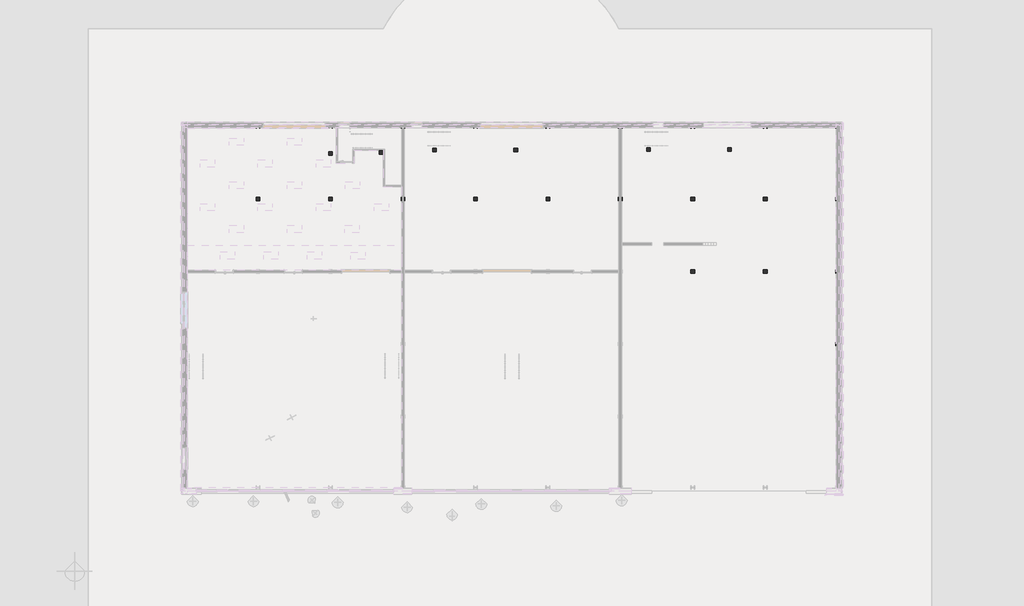
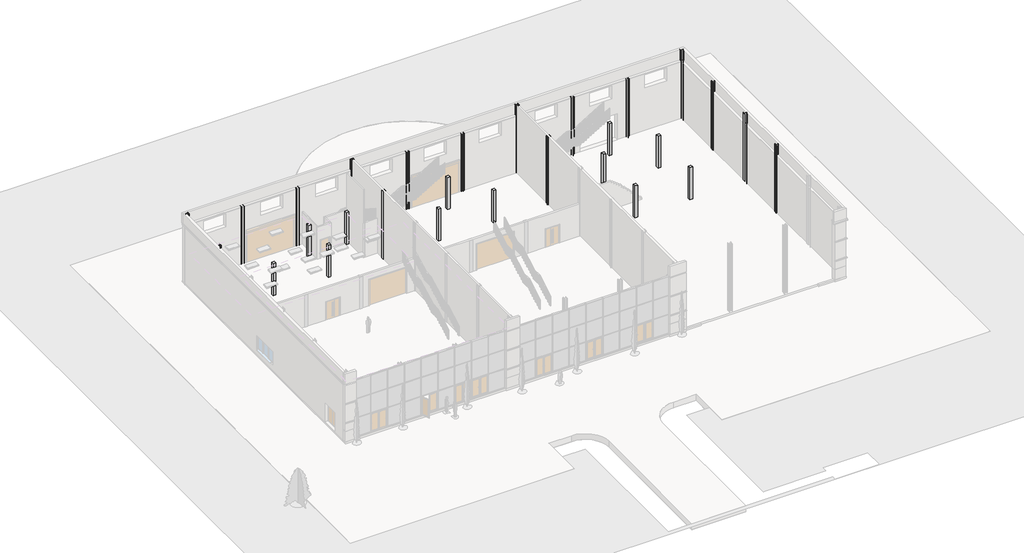
# One storey, part 6 of 13: 30 columns, 25 slabs, 2 footings.
"""IFC4 building model written with IfcOpenShell, lengths in millimetres."""

import ifcopenshell
import ifcopenshell.guid

model = None  # the IFC model being written
_history = None  # IfcOwnerHistory: only IFC2X3 demands one
_inside = {}  # id of a spatial element -> (the spatial element, [elements in it])
_under = {}  # id of a project, library or spatial element -> (it, [spatial elements below it])
_declared = {}  # id of a project -> (the project, [libraries it declares])
_typed = {}  # id of a type object -> (the type object, [elements of that type])
_made_of = {}  # id of a material, layer set ... -> (it, [elements and type objects made of it])


def new_model(schema):
    """Start an empty IFC model of exactly this schema.

    Asked for "IFC4X3", IfcOpenShell would pick the latest addendum, in which some entities
    have other attributes; the version numbers below select the first issue.
    IFC2X3 requires an IfcOwnerHistory on every rooted entity: one is made here for all.
    """
    global model, _history
    if schema == "IFC4X3":
        model = ifcopenshell.file(schema_version=(4, 3, 0, 0))
    else:
        model = ifcopenshell.file(schema=schema)
    _inside.clear()
    _under.clear()
    _declared.clear()
    _typed.clear()
    _made_of.clear()
    _history = None
    if model.schema == "IFC2X3":
        org = make("IfcOrganization", Name="unknown")
        user = make(
            "IfcPersonAndOrganization",
            ThePerson=make("IfcPerson", FamilyName="unknown"),
            TheOrganization=org,
        )
        app = make(
            "IfcApplication",
            ApplicationDeveloper=org,
            Version="unknown",
            ApplicationFullName="unknown",
            ApplicationIdentifier="unknown",
        )
        _history = make(
            "IfcOwnerHistory",
            OwningUser=user,
            OwningApplication=app,
            ChangeAction="ADDED",
            CreationDate=0,
        )
    return model


def make(cls, **values):
    """One entity of the class cls with the attributes given. An attribute that is None is left unset."""
    return model.create_entity(
        cls, **{name: value for name, value in values.items() if value is not None}
    )


def rooted(cls, **values):
    """An entity with a GlobalId (a new one), such as an element, a storey or a relation."""
    return make(cls, GlobalId=ifcopenshell.guid.new(), OwnerHistory=_history, **values)


def si_unit(unit_type, name, prefix=None):
    """IfcSIUnit, for example si_unit("LENGTHUNIT", "METRE", prefix="MILLI")."""
    return make("IfcSIUnit", UnitType=unit_type, Prefix=prefix, Name=name)


def assignment(units):
    """IfcUnitAssignment: the units of a project."""
    return None if units is None else make("IfcUnitAssignment", Units=units)


def point(xyz):
    """IfcCartesianPoint."""
    return None if xyz is None else make("IfcCartesianPoint", Coordinates=xyz)


def direction(xyz):
    """IfcDirection."""
    return None if xyz is None else make("IfcDirection", DirectionRatios=xyz)


def frame(location, z_axis=None, x_axis=None):
    """IfcAxis2Placement3D, a coordinate frame: its origin and axes. An axis left out is left unset."""
    return make(
        "IfcAxis2Placement3D",
        Location=point(location),
        Axis=direction(z_axis),
        RefDirection=direction(x_axis),
    )


def frame_2d(location, x_axis=None):
    """IfcAxis2Placement2D, a coordinate frame in the plane: its origin and x axis."""
    return make(
        "IfcAxis2Placement2D", Location=point(location), RefDirection=direction(x_axis)
    )


def origin():
    """The frame at (0, 0, 0) with its axes left unset."""
    return frame((0.0, 0.0, 0.0))


def place(relative_to, where):
    """IfcLocalPlacement: puts the frame where relative to a parent placement (None: the world)."""
    return make(
        "IfcLocalPlacement", PlacementRelTo=relative_to, RelativePlacement=where
    )


def context(
    kind, dimensions, precision=None, world=None, true_north=None, identifier=None
):
    """IfcGeometricRepresentationContext, for example the 3D "Model" context."""
    return make(
        "IfcGeometricRepresentationContext",
        ContextIdentifier=identifier,
        ContextType=kind,
        CoordinateSpaceDimension=dimensions,
        Precision=precision,
        WorldCoordinateSystem=world,
        TrueNorth=true_north,
    )


def project(units=None, contexts=None):
    """IfcProject with its units and contexts."""
    return rooted(
        "IfcProject",
        Name="project",
        RepresentationContexts=contexts,
        UnitsInContext=assignment(units),
    )


def spatial(cls, under=None, at=None, **own):
    """A site, building, storey or space (cls), placed at a placement, below another one or the project."""
    s = rooted(cls, ObjectPlacement=at, **own)
    if under is not None:
        _under.setdefault(under.id(), (under, []))[1].append(s)
    return s


def polyline(points):
    """IfcPolyline through the points."""
    return make("IfcPolyline", Points=[point(p) for p in points])


def circle_curve(where, radius):
    """IfcCircle in the frame where."""
    return make("IfcCircle", Position=where, Radius=radius)


def trimmed(basis, trim1, trim2, sense, master):
    """IfcTrimmedCurve: the piece of a basis curve between two trims."""
    return make(
        "IfcTrimmedCurve",
        BasisCurve=basis,
        Trim1=trim1,
        Trim2=trim2,
        SenseAgreement=sense,
        MasterRepresentation=master,
    )


def segment(curve, same_sense, transition):
    """IfcCompositeCurveSegment."""
    return make(
        "IfcCompositeCurveSegment",
        Transition=transition,
        SameSense=same_sense,
        ParentCurve=curve,
    )


def composite_curve(segments, self_intersect=None):
    """IfcCompositeCurve: segments joined end to end."""
    return make("IfcCompositeCurve", Segments=segments, SelfIntersect=self_intersect)


def outline(outer, holes=None, kind="AREA"):
    """IfcArbitraryClosedProfileDef: a profile drawn as a closed curve; with holes, ...WithVoids."""
    if holes is None:
        return make("IfcArbitraryClosedProfileDef", ProfileType=kind, OuterCurve=outer)
    return make(
        "IfcArbitraryProfileDefWithVoids",
        ProfileType=kind,
        OuterCurve=outer,
        InnerCurves=holes,
    )


def extrude(swept, where, along, depth):
    """IfcExtrudedAreaSolid: the profile swept, set in the frame where, extruded along a direction by depth."""
    return make(
        "IfcExtrudedAreaSolid",
        SweptArea=swept,
        Position=where,
        ExtrudedDirection=direction(along),
        Depth=depth,
    )


def faces_of(points, faces, orient=None, outer=None):
    """IfcFace entities. A face is a list of loops; a loop is a list of indices into points, from 0.

    orient and outer hold one flag for each loop. By default every Orientation is true, the
    first loop of a face is its IfcFaceOuterBound and the others are IfcFaceBound.
    """
    made = []
    for i, loops in enumerate(faces):
        bounds = []
        for j, loop in enumerate(loops):
            is_outer = j == 0 if outer is None else outer[i][j]
            bounds.append(
                make(
                    "IfcFaceOuterBound" if is_outer else "IfcFaceBound",
                    Bound=make("IfcPolyLoop", Polygon=[points[k] for k in loop]),
                    Orientation=True if orient is None else orient[i][j],
                )
            )
        made.append(make("IfcFace", Bounds=bounds))
    return made


def faceted_brep(points, faces, orient=None, outer=None, voids=None):
    """IfcFacetedBrep: a solid bounded by flat faces; with voids (closed shells), ...WithVoids."""
    shared = [point(p) for p in points]
    hull = make("IfcClosedShell", CfsFaces=faces_of(shared, faces, orient, outer))
    if voids is None:
        return make("IfcFacetedBrep", Outer=hull)
    return make(
        "IfcFacetedBrepWithVoids",
        Outer=hull,
        Voids=[
            make(cls, CfsFaces=faces_of(shared, fs, o, b)) for cls, fs, o, b in voids
        ],
    )


def shape(context_of_items, identifier, shape_type, items):
    """IfcShapeRepresentation: the items that make up one representation, for example the "Body"."""
    return make(
        "IfcShapeRepresentation",
        ContextOfItems=context_of_items,
        RepresentationIdentifier=identifier,
        RepresentationType=shape_type,
        Items=items,
    )


def source(mapping_origin, context_of_items, identifier, shape_type, items):
    """IfcRepresentationMap: a shape defined once, which mapped items show again and again."""
    return make(
        "IfcRepresentationMap",
        MappingOrigin=mapping_origin,
        MappedRepresentation=shape(context_of_items, identifier, shape_type, items),
    )


def transform(
    local_origin,
    x_axis=None,
    y_axis=None,
    z_axis=None,
    scale=None,
    scale2=None,
    scale3=None,
    uniform=True,
):
    """IfcCartesianTransformationOperator3D, or its non-uniform kind. x_axis, y_axis, z_axis: its Axis1, 2, 3."""
    if uniform:
        return make(
            "IfcCartesianTransformationOperator3D",
            Axis1=direction(x_axis),
            Axis2=direction(y_axis),
            LocalOrigin=point(local_origin),
            Scale=scale,
            Axis3=direction(z_axis),
        )
    return make(
        "IfcCartesianTransformationOperator3DnonUniform",
        Axis1=direction(x_axis),
        Axis2=direction(y_axis),
        LocalOrigin=point(local_origin),
        Scale=scale,
        Axis3=direction(z_axis),
        Scale2=scale2,
        Scale3=scale3,
    )


def mapped(mapping_source, mapping_target):
    """IfcMappedItem: shows the shape of a source again, moved by a transform."""
    return make(
        "IfcMappedItem", MappingSource=mapping_source, MappingTarget=mapping_target
    )


def made_of(thing, what):
    """Note that an element or type object is made of a material, layer set ...; save() writes the relation."""
    if what is not None:
        _made_of.setdefault(what.id(), (what, []))[1].append(thing)
    return thing


def element(
    cls,
    number,
    at=None,
    inside=None,
    cuts=None,
    type_object=None,
    material=None,
    context=None,
    identifier="Body",
    shape_type=None,
    held_by="IfcProductDefinitionShape",
    body=None,
    shapes=None,
    **own,
):
    """One element of the class cls, such as IfcWall. Its Tag is "e" and its number.

    at: its placement. inside: the storey or other place that contains it. cuts: it is an
    opening in that element (IfcRelVoidsElement). A single representation is given by context,
    identifier, shape_type and body (its items); several are given by shapes. held_by: the class
    of the entity that holds the representations. save() writes the other relations.
    """
    e = rooted(cls, Tag="e%d" % number, ObjectPlacement=at, **own)
    if body is not None:
        shapes = [shape(context, identifier, shape_type, body)]
    if shapes is not None:
        e.Representation = make(held_by, Representations=shapes)
    if inside is not None:
        _inside.setdefault(inside.id(), (inside, []))[1].append(e)
    if cuts is not None:
        rooted(
            "IfcRelVoidsElement", RelatingBuildingElement=cuts, RelatedOpeningElement=e
        )
    if type_object is not None:
        _typed.setdefault(type_object.id(), (type_object, []))[1].append(e)
    return made_of(e, material)


def aggregate(whole, parts):
    """IfcRelAggregates: a whole, such as a stair, and the parts it consists of."""
    return rooted("IfcRelAggregates", RelatingObject=whole, RelatedObjects=parts)


def save(model, path):
    """Write the relations noted so far, then the file.

    IfcRelAggregates (storeys below a building ...), IfcRelContainedInSpatialStructure (elements
    in a storey), IfcRelDefinesByType, IfcRelAssociatesMaterial and IfcRelDeclares: one each for
    every whole, place, type object, material and project.
    """
    for whole, parts in _under.values():
        aggregate(whole, parts)
    for where, things in _inside.values():
        rooted(
            "IfcRelContainedInSpatialStructure",
            RelatedElements=things,
            RelatingStructure=where,
        )
    for kind, things in _typed.values():
        rooted("IfcRelDefinesByType", RelatedObjects=things, RelatingType=kind)
    for what, things in _made_of.values():
        rooted("IfcRelAssociatesMaterial", RelatedObjects=things, RelatingMaterial=what)
    for by, libraries in _declared.values():
        rooted("IfcRelDeclares", RelatingContext=by, RelatedDefinitions=libraries)
    model.write(path)


def uc_universal_column_column_305x305x97uc_f4bfb62a(model_context):
    return source(origin(), model_context, "Body", "SweptSolid", [
        extrude(outline(composite_curve([segment(polyline([(152.65, 153.95), (152.65, 138.55), (20.15, 138.55)]), True, "CONTINUOUS"), segment(trimmed(circle_curve(frame_2d((20.15, 123.35)), 15.2), [point((20.15, 138.55))], [point((4.95, 123.35))], True, "CARTESIAN"), True, "CONTINUOUS"), segment(polyline([(4.95, 123.35), (4.95, -123.35)]), True, "CONTINUOUS"), segment(trimmed(circle_curve(frame_2d((20.15, -123.35)), 15.2), [point((4.95, -123.35))], [point((20.15, -138.55))], True, "CARTESIAN"), True, "CONTINUOUS"), segment(polyline([(20.15, -138.55), (152.65, -138.55), (152.65, -153.95), (-152.65, -153.95), (-152.65, -138.55), (-20.15, -138.55)]), True, "CONTINUOUS"), segment(trimmed(circle_curve(frame_2d((-20.15, -123.35)), 15.2), [point((-20.15, -138.55))], [point((-4.95, -123.35))], True, "CARTESIAN"), True, "CONTINUOUS"), segment(polyline([(-4.95, -123.35), (-4.95, 123.35)]), True, "CONTINUOUS"), segment(trimmed(circle_curve(frame_2d((-20.15, 123.35)), 15.2), [point((-4.95, 123.35))], [point((-20.15, 138.55))], True, "CARTESIAN"), True, "CONTINUOUS"), segment(polyline([(-20.15, 138.55), (-152.65, 138.55), (-152.65, 153.95), (152.65, 153.95)]), True, "CONTINUOUS")], self_intersect=False)), frame((0.0, 0.0, -1500.0), z_axis=(0.0, 0.0, 1.0), x_axis=(1.0, 0.0, 0.0)), (0.0, 0.0, 1.0), 9300.0),
    ])


def uc_universal_column_column_305x305x97uc_8da79b43(model_context):
    return source(origin(), model_context, "Body", "SweptSolid", [
        extrude(outline(composite_curve([segment(polyline([(152.65, -153.95), (-152.65, -153.95), (-152.65, -138.55), (-20.15, -138.55)]), True, "CONTINUOUS"), segment(trimmed(circle_curve(frame_2d((-20.15, -123.35)), 15.2), [point((-20.15, -138.55))], [point((-4.95, -123.35))], True, "CARTESIAN"), True, "CONTINUOUS"), segment(polyline([(-4.95, -123.35), (-4.95, 123.35)]), True, "CONTINUOUS"), segment(trimmed(circle_curve(frame_2d((-20.15, 123.35)), 15.2), [point((-4.95, 123.35))], [point((-20.15, 138.55))], True, "CARTESIAN"), True, "CONTINUOUS"), segment(polyline([(-20.15, 138.55), (-152.65, 138.55), (-152.65, 153.95), (152.65, 153.95), (152.65, 138.55), (20.15, 138.55)]), True, "CONTINUOUS"), segment(trimmed(circle_curve(frame_2d((20.15, 123.35)), 15.2), [point((20.15, 138.55))], [point((4.95, 123.35))], True, "CARTESIAN"), True, "CONTINUOUS"), segment(polyline([(4.95, 123.35), (4.95, -123.35)]), True, "CONTINUOUS"), segment(trimmed(circle_curve(frame_2d((20.15, -123.35)), 15.2), [point((4.95, -123.35))], [point((20.15, -138.55))], True, "CARTESIAN"), True, "CONTINUOUS"), segment(polyline([(20.15, -138.55), (152.65, -138.55), (152.65, -153.95)]), True, "CONTINUOUS")], self_intersect=False)), frame((0.0, 0.0, -1500.0), z_axis=(0.0, 0.0, 1.0), x_axis=(1.0, 0.0, 0.0)), (0.0, 0.0, 1.0), 9300.0),
    ])


def uc_universal_column_column_305x305x97uc_43a052ce(model_context):
    return source(origin(), model_context, "Body", "SweptSolid", [
        extrude(outline(composite_curve([segment(polyline([(152.65, 153.95), (152.65, 138.55), (20.15, 138.55)]), True, "CONTINUOUS"), segment(trimmed(circle_curve(frame_2d((20.15, 123.35)), 15.2), [point((20.15, 138.55))], [point((4.95, 123.35))], True, "CARTESIAN"), True, "CONTINUOUS"), segment(polyline([(4.95, 123.35), (4.95, -123.35)]), True, "CONTINUOUS"), segment(trimmed(circle_curve(frame_2d((20.15, -123.35)), 15.2), [point((4.95, -123.35))], [point((20.15, -138.55))], True, "CARTESIAN"), True, "CONTINUOUS"), segment(polyline([(20.15, -138.55), (152.65, -138.55), (152.65, -153.95), (-152.65, -153.95), (-152.65, -138.55), (-20.15, -138.55)]), True, "CONTINUOUS"), segment(trimmed(circle_curve(frame_2d((-20.15, -123.35)), 15.2), [point((-20.15, -138.55))], [point((-4.95, -123.35))], True, "CARTESIAN"), True, "CONTINUOUS"), segment(polyline([(-4.95, -123.35), (-4.95, 123.35)]), True, "CONTINUOUS"), segment(trimmed(circle_curve(frame_2d((-20.15, 123.35)), 15.2), [point((-4.95, 123.35))], [point((-20.15, 138.55))], True, "CARTESIAN"), True, "CONTINUOUS"), segment(polyline([(-20.15, 138.55), (-152.65, 138.55), (-152.65, 153.95), (152.65, 153.95)]), True, "CONTINUOUS")], self_intersect=False)), frame((0.0, 0.0, -1500.0), z_axis=(0.0, 0.0, 1.0), x_axis=(1.0, 0.0, 0.0)), (0.0, 0.0, 1.0), 8100.0),
    ])


def pad_foundation_rectangular_1000x1000x500_ed6229e9(model_context):
    return source(origin(), model_context, "Body", "SweptSolid", [
        extrude(outline(polyline([(500.0, 500.0), (500.0, -500.0), (-500.0, -500.0), (-500.0, 500.0), (500.0, 500.0)])), frame((0.0, 0.0, -500.0), z_axis=(0.0, 0.0, 1.0), x_axis=(1.0, 0.0, 0.0)), (0.0, 0.0, 1.0), 500.0),
    ])


model = new_model("IFC4")

# Units and contexts
model_context = context("Model", 3, world=origin())
ifc_project = project(units=[si_unit("LENGTHUNIT", "METRE", prefix="MILLI")], contexts=[model_context])

# Site, building, storey
site = spatial("IfcSite", under=ifc_project)
building = spatial("IfcBuilding", under=site)
storey = spatial("IfcBuildingStorey", under=building, Name="L0 - Ground Floor (Shadows On)", Elevation=0.0)

# Columns
placement = place(None, origin())
element("IfcColumn", 1, ObjectType="Concrete Square : 300 x 300mm", at=placement, inside=storey, context=model_context, shape_type="SweptSolid", body=[
    extrude(outline(polyline([(-989.5553457, 791.2380918), (-1289.5553457, 791.2380918), (-1289.5553457, 1091.2380918), (-989.5553457, 1091.2380918), (-989.5553457, 791.2380918)])), frame((0.0, 0.0, -1500.0), z_axis=(0.0, 0.0, 1.0), x_axis=(1.0, 0.0, 0.0)), (0.0, 0.0, 1.0), 5200.0),
])
element("IfcColumn", 2, ObjectType="Concrete Square : 300 x 300mm", at=placement, inside=storey, context=model_context, shape_type="SweptSolid", body=[
    extrude(outline(polyline([(9194.5066977, 4635.3001351), (8894.5066977, 4635.3001351), (8894.5066977, 4935.3001351), (9194.5066977, 4935.3001351), (9194.5066977, 4635.3001351)])), frame((0.0, 0.0, -1500.0), z_axis=(0.0, 0.0, 1.0), x_axis=(1.0, 0.0, 0.0)), (0.0, 0.0, 1.0), 5200.0),
])
element("IfcColumn", 3, ObjectType="Concrete Square : 300 x 300mm", at=placement, inside=storey, context=model_context, shape_type="SweptSolid", body=[
    extrude(outline(polyline([(17010.4446543, 791.2380918), (16710.4446543, 791.2380918), (16710.4446543, 1091.2380918), (17010.4446543, 1091.2380918), (17010.4446543, 791.2380918)])), frame((0.0, 0.0, -1500.0), z_axis=(0.0, 0.0, 1.0), x_axis=(1.0, 0.0, 0.0)), (0.0, 0.0, 1.0), 5200.0),
])
element("IfcColumn", 4, ObjectType="Concrete Square : 300 x 300mm", at=placement, inside=storey, context=model_context, shape_type="SweptSolid", body=[
    extrude(outline(polyline([(23010.4446543, 791.2380918), (22710.4446543, 791.2380918), (22710.4446543, 1091.2380918), (23010.4446543, 1091.2380918), (23010.4446543, 791.2380918)])), frame((0.0, 0.0, -1500.0), z_axis=(0.0, 0.0, 1.0), x_axis=(1.0, 0.0, 0.0)), (0.0, 0.0, 1.0), 5200.0),
])
element("IfcColumn", 5, ObjectType="Concrete Square : 300 x 300mm", at=placement, inside=storey, context=model_context, shape_type="SweptSolid", body=[
    extrude(outline(polyline([(35010.4446543, 791.2380918), (34710.4446543, 791.2380918), (34710.4446543, 1091.2380918), (35010.4446543, 1091.2380918), (35010.4446543, 791.2380918)])), frame((0.0, 0.0, -1500.0), z_axis=(0.0, 0.0, 1.0), x_axis=(1.0, 0.0, 0.0)), (0.0, 0.0, 1.0), 5200.0),
])
element("IfcColumn", 6, ObjectType="Concrete Square : 300 x 300mm", at=placement, inside=storey, context=model_context, shape_type="SweptSolid", body=[
    extrude(outline(polyline([(41010.4446543, 791.2380918), (40710.4446543, 791.2380918), (40710.4446543, 1091.2380918), (41010.4446543, 1091.2380918), (41010.4446543, 791.2380918)])), frame((0.0, 0.0, -1500.0), z_axis=(0.0, 0.0, 1.0), x_axis=(1.0, 0.0, 0.0)), (0.0, 0.0, 1.0), 5200.0),
])
element("IfcColumn", 7, ObjectType="Concrete Square : 300 x 300mm", at=placement, inside=storey, context=model_context, shape_type="SweptSolid", body=[
    extrude(outline(polyline([(35010.4446543, -5208.7619082), (34710.4446543, -5208.7619082), (34710.4446543, -4908.7619082), (35010.4446543, -4908.7619082), (35010.4446543, -5208.7619082)])), frame((0.0, 0.0, -1500.0), z_axis=(0.0, 0.0, 1.0), x_axis=(1.0, 0.0, 0.0)), (0.0, 0.0, 1.0), 5200.0),
])
element("IfcColumn", 8, ObjectType="Concrete Square : 300 x 300mm", at=placement, inside=storey, context=model_context, shape_type="SweptSolid", body=[
    extrude(outline(polyline([(41010.4446543, -5208.7619082), (40710.4446543, -5208.7619082), (40710.4446543, -4908.7619082), (41010.4446543, -4908.7619082), (41010.4446543, -5208.7619082)])), frame((0.0, 0.0, -1500.0), z_axis=(0.0, 0.0, 1.0), x_axis=(1.0, 0.0, 0.0)), (0.0, 0.0, 1.0), 5200.0),
])
element("IfcColumn", 9, ObjectType="Concrete Square : 300 x 300mm", at=placement, inside=storey, context=model_context, shape_type="SweptSolid", body=[
    extrude(outline(polyline([(5010.4446543, 791.2380918), (4710.4446543, 791.2380918), (4710.4446543, 1091.2380918), (5010.4446543, 1091.2380918), (5010.4446543, 791.2380918)])), frame((0.0, 0.0, -1500.0), z_axis=(0.0, 0.0, 1.0), x_axis=(1.0, 0.0, 0.0)), (0.0, 0.0, 1.0), 5200.0),
])
element("IfcColumn", 10, ObjectType="Concrete Square : 300 x 300mm", at=placement, inside=storey, context=model_context, shape_type="SweptSolid", body=[
    extrude(outline(polyline([(5022.9446543, 4575.3001351), (4722.9446543, 4575.3001351), (4722.9446543, 4875.3001351), (5022.9446543, 4875.3001351), (5022.9446543, 4575.3001351)])), frame((0.0, 0.0, -1500.0), z_axis=(0.0, 0.0, 1.0), x_axis=(1.0, 0.0, 0.0)), (0.0, 0.0, 1.0), 5200.0),
])
element("IfcColumn", 11, ObjectType="Concrete Square : 300 x 300mm", at=placement, inside=storey, context=model_context, shape_type="SweptSolid", body=[
    extrude(outline(polyline([(20350.4446543, 4850.3001351), (20050.4446543, 4850.3001351), (20050.4446543, 5150.3001351), (20350.4446543, 5150.3001351), (20350.4446543, 4850.3001351)])), frame((0.0, 0.0, -1500.0), z_axis=(0.0, 0.0, 1.0), x_axis=(1.0, 0.0, 0.0)), (0.0, 0.0, 1.0), 5200.0),
])
element("IfcColumn", 12, ObjectType="Concrete Square : 300 x 300mm", at=placement, inside=storey, context=model_context, shape_type="SweptSolid", body=[
    extrude(outline(polyline([(13627.9446543, 5150.3001351), (13627.9446543, 4850.3001351), (13327.9446543, 4850.3001351), (13327.9446543, 5150.3001351), (13627.9446543, 5150.3001351)])), frame((0.0, 0.0, -1500.0), z_axis=(0.0, 0.0, 1.0), x_axis=(1.0, 0.0, 0.0)), (0.0, 0.0, 1.0), 5200.0),
])
element("IfcColumn", 13, ObjectType="Concrete Square : 300 x 300mm", at=placement, inside=storey, context=model_context, shape_type="SweptSolid", body=[
    extrude(outline(polyline([(31350.4446543, 4891.2380918), (31050.4446543, 4891.2380918), (31050.4446543, 5191.2380918), (31350.4446543, 5191.2380918), (31350.4446543, 4891.2380918)])), frame((0.0, 0.0, -1500.0), z_axis=(0.0, 0.0, 1.0), x_axis=(1.0, 0.0, 0.0)), (0.0, 0.0, 1.0), 5200.0),
])
element("IfcColumn", 14, ObjectType="Concrete Square : 300 x 300mm", at=placement, inside=storey, context=model_context, shape_type="SweptSolid", body=[
    extrude(outline(polyline([(38050.4446543, 4891.2380918), (37750.4446543, 4891.2380918), (37750.4446543, 5191.2380918), (38050.4446543, 5191.2380918), (38050.4446543, 4891.2380918)])), frame((0.0, 0.0, -1500.0), z_axis=(0.0, 0.0, 1.0), x_axis=(1.0, 0.0, 0.0)), (0.0, 0.0, 1.0), 5200.0),
])
element("IfcColumn", 15, ObjectType="UC-Universal Column-Column : 305x305x97UC", at=placement, inside=storey, context=model_context, shape_type="SweptSolid", body=[
    extrude(outline(composite_curve([segment(polyline([(-7293.5053457, 1093.8880918), (-7278.1053457, 1093.8880918), (-7278.1053457, 961.3880918)]), True, "CONTINUOUS"), segment(trimmed(circle_curve(frame_2d((-7262.9053457, 961.3880918)), 15.2), [point((-7278.1053457, 961.3880918))], [point((-7262.9053457, 946.1880918))], True, "CARTESIAN"), True, "CONTINUOUS"), segment(polyline([(-7262.9053457, 946.1880918), (-7016.2053457, 946.1880918)]), True, "CONTINUOUS"), segment(trimmed(circle_curve(frame_2d((-7016.2053457, 961.3880918)), 15.2), [point((-7016.2053457, 946.1880918))], [point((-7001.0053457, 961.3880918))], True, "CARTESIAN"), True, "CONTINUOUS"), segment(polyline([(-7001.0053457, 961.3880918), (-7001.0053457, 1093.8880918), (-6985.6053457, 1093.8880918), (-6985.6053457, 788.5880918), (-7001.0053457, 788.5880918), (-7001.0053457, 921.0880918)]), True, "CONTINUOUS"), segment(trimmed(circle_curve(frame_2d((-7016.2053457, 921.0880918)), 15.2), [point((-7001.0053457, 921.0880918))], [point((-7016.2053457, 936.2880918))], True, "CARTESIAN"), True, "CONTINUOUS"), segment(polyline([(-7016.2053457, 936.2880918), (-7262.9053457, 936.2880918)]), True, "CONTINUOUS"), segment(trimmed(circle_curve(frame_2d((-7262.9053457, 921.0880918)), 15.2), [point((-7262.9053457, 936.2880918))], [point((-7278.1053457, 921.0880918))], True, "CARTESIAN"), True, "CONTINUOUS"), segment(polyline([(-7278.1053457, 921.0880918), (-7278.1053457, 788.5880918), (-7293.5053457, 788.5880918), (-7293.5053457, 1093.8880918)]), True, "CONTINUOUS")], self_intersect=False)), frame((0.0, 0.0, -1500.0), z_axis=(0.0, 0.0, 1.0), x_axis=(1.0, 0.0, 0.0)), (0.0, 0.0, 1.0), 9300.0),
])
uc_universal_column_column_305x305x97uc_shape = uc_universal_column_column_305x305x97uc_f4bfb62a(model_context)
element("IfcColumn", 16, ObjectType="UC-Universal Column-Column : 305x305x97UC", at=placement, inside=storey, context=model_context, shape_type="MappedRepresentation", body=[
    mapped(uc_universal_column_column_305x305x97uc_shape, transform((-7139.5553457, 6941.2380918, 0.0), x_axis=(0.0, 1.0, 0.0), y_axis=(-1.0, 0.0, 0.0), z_axis=(0.0, 0.0, 1.0))),
])
element("IfcColumn", 17, ObjectType="UC-Universal Column-Column : 305x305x97UC", at=placement, inside=storey, context=model_context, shape_type="MappedRepresentation", body=[
    mapped(uc_universal_column_column_305x305x97uc_shape, transform((10860.4446543, 6941.2380918, 0.0), x_axis=(0.0, 1.0, 0.0), y_axis=(-1.0, 0.0, 0.0), z_axis=(0.0, 0.0, 1.0))),
])
element("IfcColumn", 18, ObjectType="UC-Universal Column-Column : 305x305x97UC", at=placement, inside=storey, context=model_context, shape_type="MappedRepresentation", body=[
    mapped(uc_universal_column_column_305x305x97uc_shape, transform((28860.4446543, 6941.2380918, 0.0), x_axis=(0.0, 1.0, 0.0), y_axis=(-1.0, 0.0, 0.0), z_axis=(0.0, 0.0, 1.0))),
])
element("IfcColumn", 19, ObjectType="UC-Universal Column-Column : 305x305x97UC", at=placement, inside=storey, context=model_context, shape_type="MappedRepresentation", body=[
    mapped(uc_universal_column_column_305x305x97uc_shape, transform((10860.4446543, 941.2380918, 0.0), x_axis=(0.0, 1.0, 0.0), y_axis=(-1.0, 0.0, 0.0), z_axis=(0.0, 0.0, 1.0))),
])
element("IfcColumn", 20, ObjectType="UC-Universal Column-Column : 305x305x97UC", at=placement, inside=storey, context=model_context, shape_type="MappedRepresentation", body=[
    mapped(uc_universal_column_column_305x305x97uc_shape, transform((28860.4446543, 941.2380918, 0.0), x_axis=(0.0, 1.0, 0.0), y_axis=(-1.0, 0.0, 0.0), z_axis=(0.0, 0.0, 1.0))),
])
uc_universal_column_column_305x305x97uc_2_shape = uc_universal_column_column_305x305x97uc_8da79b43(model_context)
element("IfcColumn", 21, ObjectType="UC-Universal Column-Column : 305x305x97UC", at=placement, inside=storey, context=model_context, shape_type="MappedRepresentation", body=[
    mapped(uc_universal_column_column_305x305x97uc_2_shape, transform((46860.4446543, -11058.7619082, 0.0), x_axis=(0.0, 1.0, 0.0), y_axis=(-1.0, 0.0, 0.0), z_axis=(0.0, 0.0, 1.0))),
])
element("IfcColumn", 22, ObjectType="UC-Universal Column-Column : 305x305x97UC", at=placement, inside=storey, context=model_context, shape_type="MappedRepresentation", body=[
    mapped(uc_universal_column_column_305x305x97uc_2_shape, transform((46860.4446543, -5058.7619082, 0.0), x_axis=(0.0, 1.0, 0.0), y_axis=(-1.0, 0.0, 0.0), z_axis=(0.0, 0.0, 1.0))),
])
element("IfcColumn", 23, ObjectType="UC-Universal Column-Column : 305x305x97UC", at=placement, inside=storey, context=model_context, shape_type="MappedRepresentation", body=[
    mapped(uc_universal_column_column_305x305x97uc_2_shape, transform((46860.4446543, 941.2380918, 0.0), x_axis=(0.0, 1.0, 0.0), y_axis=(-1.0, 0.0, 0.0), z_axis=(0.0, 0.0, 1.0))),
])
element("IfcColumn", 24, ObjectType="UC-Universal Column-Column : 305x305x97UC", at=placement, inside=storey, context=model_context, shape_type="MappedRepresentation", body=[
    mapped(uc_universal_column_column_305x305x97uc_2_shape, transform((46860.4446543, 6941.2380918, 0.0), x_axis=(0.0, 1.0, 0.0), y_axis=(-1.0, 0.0, 0.0), z_axis=(0.0, 0.0, 1.0))),
])
uc_universal_column_column_305x305x97uc_3_shape = uc_universal_column_column_305x305x97uc_43a052ce(model_context)
element("IfcColumn", 25, ObjectType="UC-Universal Column-Column : 305x305x97UC", at=placement, inside=storey, context=model_context, shape_type="MappedRepresentation", body=[
    mapped(uc_universal_column_column_305x305x97uc_3_shape, transform((-1139.5553457, 6941.2380918, 0.0), x_axis=(0.0, 1.0, 0.0), y_axis=(-1.0, 0.0, 0.0), z_axis=(0.0, 0.0, 1.0))),
])
element("IfcColumn", 26, ObjectType="UC-Universal Column-Column : 305x305x97UC", at=placement, inside=storey, context=model_context, shape_type="MappedRepresentation", body=[
    mapped(uc_universal_column_column_305x305x97uc_3_shape, transform((4860.4446543, 6941.2380918, 0.0), x_axis=(0.0, 1.0, 0.0), y_axis=(-1.0, 0.0, 0.0), z_axis=(0.0, 0.0, 1.0))),
])
element("IfcColumn", 27, ObjectType="UC-Universal Column-Column : 305x305x97UC", at=placement, inside=storey, context=model_context, shape_type="MappedRepresentation", body=[
    mapped(uc_universal_column_column_305x305x97uc_3_shape, transform((16860.4446543, 6941.2380918, 0.0), x_axis=(0.0, 1.0, 0.0), y_axis=(-1.0, 0.0, 0.0), z_axis=(0.0, 0.0, 1.0))),
])
element("IfcColumn", 28, ObjectType="UC-Universal Column-Column : 305x305x97UC", at=placement, inside=storey, context=model_context, shape_type="MappedRepresentation", body=[
    mapped(uc_universal_column_column_305x305x97uc_3_shape, transform((22860.4446543, 6941.2380918, 0.0), x_axis=(0.0, 1.0, 0.0), y_axis=(-1.0, 0.0, 0.0), z_axis=(0.0, 0.0, 1.0))),
])
element("IfcColumn", 29, ObjectType="UC-Universal Column-Column : 305x305x97UC", at=placement, inside=storey, context=model_context, shape_type="MappedRepresentation", body=[
    mapped(uc_universal_column_column_305x305x97uc_3_shape, transform((34860.4446543, 6941.2380918, 0.0), x_axis=(0.0, 1.0, 0.0), y_axis=(-1.0, 0.0, 0.0), z_axis=(0.0, 0.0, 1.0))),
])
element("IfcColumn", 30, ObjectType="UC-Universal Column-Column : 305x305x97UC", at=placement, inside=storey, context=model_context, shape_type="MappedRepresentation", body=[
    mapped(uc_universal_column_column_305x305x97uc_3_shape, transform((40860.4446543, 6941.2380918, 0.0), x_axis=(0.0, 1.0, 0.0), y_axis=(-1.0, 0.0, 0.0), z_axis=(0.0, 0.0, 1.0))),
])

# Footings
element("IfcFooting", 31, ObjectType="Wall Foundation - Commercial 1300 x 450", at=placement, inside=storey, context=model_context, shape_type="Brep", body=[
    faceted_brep([(47425.1446543, 7505.9380918, -1200.0), (46510.7446543, 7505.9380918, -1200.0), (46510.7446543, 6591.5380918, -1200.0), (46510.7446543, -22819.0474846, -1200.0), (47425.1446543, -22819.0474846, -1200.0), (47425.1446543, 7505.9380918, -1504.8), (47425.1446543, -22819.0474846, -1504.8), (46510.7446543, 7505.9380918, -1504.8), (47360.4446543, -22819.0474846, -1504.8), (47360.4446543, -22448.7619082, -1504.8), (46510.7446543, -22448.7619082, -1504.8), (46510.7446543, -17558.7619082, -1504.8), (47360.4446543, -17558.7619082, -1504.8), (47360.4446543, -16558.7619082, -1504.8), (46510.7446543, -16558.7619082, -1504.8), (46510.7446543, -11558.7619082, -1504.8), (47360.4446543, -11558.7619082, -1504.8), (47360.4446543, -10558.7619082, -1504.8), (46510.7446543, -10558.7619082, -1504.8), (46510.7446543, -5558.7619082, -1504.8), (47360.4446543, -5558.7619082, -1504.8), (47360.4446543, -4558.7619082, -1504.8), (46510.7446543, -4558.7619082, -1504.8), (46510.7446543, 441.2380918, -1504.8), (47360.4446543, 441.2380918, -1504.8), (47360.4446543, 1441.2380918, -1504.8), (46510.7446543, 1441.2380918, -1504.8), (46510.7446543, 6441.2380918, -1504.8), (47360.4446543, 6441.2380918, -1504.8), (47360.4446543, 7441.2380918, -1504.8), (46510.7446543, 7441.2380918, -1504.8), (46510.7446543, 7441.2380918, -1500.0), (46510.7446543, 6591.5380918, -1500.0), (46510.7446543, 6441.2380918, -1500.0), (46510.7446543, 1441.2380918, -1500.0), (46510.7446543, 441.2380918, -1500.0), (46510.7446543, -4558.7619082, -1500.0), (46510.7446543, -5558.7619082, -1500.0), (46510.7446543, -10558.7619082, -1500.0), (46510.7446543, -11558.7619082, -1500.0), (46510.7446543, -16558.7619082, -1500.0), (46510.7446543, -17558.7619082, -1500.0), (46510.7446543, -22448.7619082, -1500.0), (46510.7446543, -22819.0474846, -1500.0), (47360.4446543, 1441.2380918, -1500.0), (47360.4446543, 441.2380918, -1500.0), (47360.4446543, 7441.2380918, -1500.0), (47360.4446543, 6441.2380918, -1500.0), (47360.4446543, -4558.7619082, -1500.0), (47360.4446543, -5558.7619082, -1500.0), (47360.4446543, -10558.7619082, -1500.0), (47360.4446543, -11558.7619082, -1500.0), (47360.4446543, -16558.7619082, -1500.0), (47360.4446543, -17558.7619082, -1500.0), (47360.4446543, -22448.7619082, -1500.0), (47360.4446543, -22819.0474846, -1500.0)], [[[0, 1, 2, 3, 4]], [[5, 0, 4, 6]], [[7, 5, 6, 8, 9, 10, 11, 12, 13, 14, 15, 16, 17, 18, 19, 20, 21, 22, 23, 24, 25, 26, 27, 28, 29, 30]], [[1, 7, 30, 31, 32, 33, 27, 26, 34, 35, 23, 22, 36, 37, 19, 18, 38, 39, 15, 14, 40, 41, 11, 10, 42, 43, 3, 2]], [[1, 0, 5, 7]], [[44, 45, 35, 34]], [[44, 34, 26, 25]], [[35, 45, 24, 23]], [[45, 44, 25, 24]], [[46, 47, 33, 32, 31]], [[33, 47, 28, 27]], [[47, 46, 29, 28]], [[48, 49, 37, 36]], [[48, 36, 22, 21]], [[37, 49, 20, 19]], [[49, 48, 21, 20]], [[50, 51, 39, 38]], [[50, 38, 18, 17]], [[39, 51, 16, 15]], [[51, 50, 17, 16]], [[52, 53, 41, 40]], [[52, 40, 14, 13]], [[41, 53, 12, 11]], [[53, 52, 13, 12]], [[42, 54, 55, 43]], [[54, 42, 10, 9]], [[54, 9, 8, 55]], [[4, 3, 43, 55, 8, 6]], [[46, 31, 30, 29]]]),
])
element("IfcFooting", 32, ObjectType="Wall Foundation - Commercial 1300 x 450", at=placement, inside=storey, context=model_context, shape_type="Brep", body=[
    faceted_brep([(46510.7446543, 6591.5380918, -1200.0), (46510.7446543, 7505.9380918, -1200.0), (-6758.8053457, 7505.9380918, -1200.0), (-6758.8053457, 6591.5380918, -1200.0), (10403.2446543, 6591.5380918, -1200.0), (11317.6446543, 6591.5380918, -1200.0), (28403.2446543, 6591.5380918, -1200.0), (29317.6446543, 6591.5380918, -1200.0), (46510.7446543, 7505.9380918, -1504.8), (-6758.8053457, 7505.9380918, -1504.8), (41386.4946543, 7441.2380918, -1504.8), (40386.4946543, 7441.2380918, -1504.8), (40386.4946543, 6591.5380918, -1504.8), (35347.9446543, 6591.5380918, -1504.8), (35347.9446543, 7441.2380918, -1504.8), (34347.9446543, 7441.2380918, -1504.8), (34347.9446543, 6591.5380918, -1504.8), (29360.4446543, 6591.5380918, -1504.8), (29360.4446543, 7441.2380918, -1504.8), (28360.4446543, 7441.2380918, -1504.8), (28360.4446543, 6591.5380918, -1504.8), (23360.4446543, 6591.5380918, -1504.8), (23360.4446543, 7441.2380918, -1504.8), (22360.4446543, 7441.2380918, -1504.8), (22360.4446543, 6591.5380918, -1504.8), (17360.4446543, 6591.5380918, -1504.8), (17360.4446543, 7441.2380918, -1504.8), (16360.4446543, 7441.2380918, -1504.8), (16360.4446543, 6591.5380918, -1504.8), (11360.4446543, 6591.5380918, -1504.8), (11360.4446543, 7441.2380918, -1504.8), (10360.4446543, 7441.2380918, -1504.8), (10360.4446543, 6591.5380918, -1504.8), (5360.4446543, 6591.5380918, -1504.8), (5360.4446543, 7441.2380918, -1504.8), (4360.4446543, 7441.2380918, -1504.8), (4360.4446543, 6591.5380918, -1504.8), (-639.5553457, 6591.5380918, -1504.8), (-639.5553457, 7441.2380918, -1504.8), (-1639.5553457, 7441.2380918, -1504.8), (-1639.5553457, 6591.5380918, -1504.8), (-6639.5553457, 6591.5380918, -1504.8), (-6639.5553457, 7441.2380918, -1504.8), (-6758.8053457, 7441.2380918, -1504.8), (46510.7446543, 7441.2380918, -1504.8), (46360.4446543, 7441.2380918, -1504.8), (46360.4446543, 6591.5380918, -1504.8), (41386.4946543, 6591.5380918, -1504.8), (40386.4946543, 6591.5380918, -1500.0), (41386.4946543, 6591.5380918, -1500.0), (46360.4446543, 6591.5380918, -1500.0), (46510.7446543, 6591.5380918, -1500.0), (-6758.8053457, 6591.5380918, -1500.0), (-6639.5553457, 6591.5380918, -1500.0), (-1639.5553457, 6591.5380918, -1500.0), (-639.5553457, 6591.5380918, -1500.0), (4360.4446543, 6591.5380918, -1500.0), (5360.4446543, 6591.5380918, -1500.0), (10360.4446543, 6591.5380918, -1500.0), (10403.2446543, 6591.5380918, -1500.0), (11317.6446543, 6591.5380918, -1500.0), (11360.4446543, 6591.5380918, -1500.0), (16360.4446543, 6591.5380918, -1500.0), (17360.4446543, 6591.5380918, -1500.0), (22360.4446543, 6591.5380918, -1500.0), (23360.4446543, 6591.5380918, -1500.0), (28360.4446543, 6591.5380918, -1500.0), (28403.2446543, 6591.5380918, -1500.0), (29317.6446543, 6591.5380918, -1500.0), (29360.4446543, 6591.5380918, -1500.0), (34347.9446543, 6591.5380918, -1500.0), (35347.9446543, 6591.5380918, -1500.0), (40386.4946543, 7441.2380918, -1500.0), (41386.4946543, 7441.2380918, -1500.0), (34347.9446543, 7441.2380918, -1500.0), (35347.9446543, 7441.2380918, -1500.0), (28360.4446543, 7441.2380918, -1500.0), (29360.4446543, 7441.2380918, -1500.0), (22360.4446543, 7441.2380918, -1500.0), (23360.4446543, 7441.2380918, -1500.0), (16360.4446543, 7441.2380918, -1500.0), (17360.4446543, 7441.2380918, -1500.0), (10360.4446543, 7441.2380918, -1500.0), (11360.4446543, 7441.2380918, -1500.0), (4360.4446543, 7441.2380918, -1500.0), (5360.4446543, 7441.2380918, -1500.0), (-1639.5553457, 7441.2380918, -1500.0), (-639.5553457, 7441.2380918, -1500.0), (-6639.5553457, 7441.2380918, -1500.0), (-6758.8053457, 7441.2380918, -1500.0), (46510.7446543, 7441.2380918, -1500.0), (46360.4446543, 7441.2380918, -1500.0)], [[[0, 1, 2, 3, 4, 5, 6, 7]], [[1, 8, 9, 2]], [[10, 11, 12, 13, 14, 15, 16, 17, 18, 19, 20, 21, 22, 23, 24, 25, 26, 27, 28, 29, 30, 31, 32, 33, 34, 35, 36, 37, 38, 39, 40, 41, 42, 43, 9, 8, 44, 45, 46, 47]], [[48, 49, 47, 46, 50, 51, 0, 7, 6, 5, 4, 3, 52, 53, 41, 40, 54, 55, 37, 36, 56, 57, 33, 32, 58, 59, 60, 61, 29, 28, 62, 63, 25, 24, 64, 65, 21, 20, 66, 67, 68, 69, 17, 16, 70, 71, 13, 12]], [[72, 73, 49, 48]], [[73, 72, 11, 10]], [[72, 48, 12, 11]], [[49, 73, 10, 47]], [[74, 75, 71, 70]], [[75, 74, 15, 14]], [[74, 70, 16, 15]], [[71, 75, 14, 13]], [[76, 77, 69, 68, 67, 66]], [[77, 76, 19, 18]], [[76, 66, 20, 19]], [[69, 77, 18, 17]], [[78, 79, 65, 64]], [[79, 78, 23, 22]], [[78, 64, 24, 23]], [[65, 79, 22, 21]], [[80, 81, 63, 62]], [[81, 80, 27, 26]], [[80, 62, 28, 27]], [[63, 81, 26, 25]], [[82, 83, 61, 60, 59, 58]], [[83, 82, 31, 30]], [[82, 58, 32, 31]], [[61, 83, 30, 29]], [[84, 85, 57, 56]], [[85, 84, 35, 34]], [[84, 56, 36, 35]], [[57, 85, 34, 33]], [[86, 87, 55, 54]], [[87, 86, 39, 38]], [[86, 54, 40, 39]], [[55, 87, 38, 37]], [[88, 53, 52, 89]], [[42, 88, 89, 43]], [[53, 88, 42, 41]], [[52, 3, 2, 9, 43, 89]], [[1, 0, 51, 90, 44, 8]], [[50, 91, 90, 51]], [[90, 91, 45, 44]], [[91, 50, 46, 45]]]),
])

# Slabs
element("IfcSlab", 33, ObjectType="Pad Foundation-Rectangular : 1000x1000x500", at=placement, inside=storey, context=model_context, shape_type="Brep", body=[
    faceted_brep([(11360.4446543, 1441.2380918, -1500.0), (11317.6446543, 1441.2380918, -1500.0), (10403.2446543, 1441.2380918, -1500.0), (10360.4446543, 1441.2380918, -1500.0), (10360.4446543, 441.2380918, -1500.0), (10403.2446543, 441.2380918, -1500.0), (11317.6446543, 441.2380918, -1500.0), (11360.4446543, 441.2380918, -1500.0), (11360.4446543, 1441.2380918, -2000.0), (11360.4446543, 441.2380918, -2000.0), (10360.4446543, 441.2380918, -2000.0), (10360.4446543, 1441.2380918, -2000.0)], [[[0, 1, 2, 3, 4, 5, 6, 7]], [[8, 9, 10, 11]], [[3, 2, 1, 0, 8, 11]], [[4, 3, 11, 10]], [[7, 6, 5, 4, 10, 9]], [[0, 7, 9, 8]]]),
])
element("IfcSlab", 34, ObjectType="Pad Foundation-Rectangular : 1000x1000x500", at=placement, inside=storey, context=model_context, shape_type="Brep", body=[
    faceted_brep([(29360.4446543, 1441.2380918, -1500.0), (29317.6446543, 1441.2380918, -1500.0), (28403.2446543, 1441.2380918, -1500.0), (28360.4446543, 1441.2380918, -1500.0), (28360.4446543, 441.2380918, -1500.0), (28403.2446543, 441.2380918, -1500.0), (29317.6446543, 441.2380918, -1500.0), (29360.4446543, 441.2380918, -1500.0), (29360.4446543, 1441.2380918, -2000.0), (29360.4446543, 441.2380918, -2000.0), (28360.4446543, 441.2380918, -2000.0), (28360.4446543, 1441.2380918, -2000.0)], [[[0, 1, 2, 3, 4, 5, 6, 7]], [[8, 9, 10, 11]], [[3, 2, 1, 0, 8, 11]], [[4, 3, 11, 10]], [[7, 6, 5, 4, 10, 9]], [[0, 7, 9, 8]]]),
])
element("IfcSlab", 35, ObjectType="Pad Foundation-Rectangular : 1000x1000x500", at=placement, inside=storey, context=model_context, shape_type="Brep", body=[
    faceted_brep([(41386.4946543, 7441.2380918, -1500.0), (40386.4946543, 7441.2380918, -1500.0), (40386.4946543, 6591.5380918, -1500.0), (40386.4946543, 6441.2380918, -1500.0), (41386.4946543, 6441.2380918, -1500.0), (41386.4946543, 6591.5380918, -1500.0), (41386.4946543, 7441.2380918, -2000.0), (41386.4946543, 6441.2380918, -2000.0), (40386.4946543, 6441.2380918, -2000.0), (40386.4946543, 7441.2380918, -2000.0), (41386.4946543, 7441.2380918, -1504.8), (40386.4946543, 7441.2380918, -1504.8)], [[[0, 1, 2, 3, 4, 5]], [[6, 7, 8, 9]], [[1, 0, 10, 6, 9, 11]], [[3, 2, 1, 11, 9, 8]], [[4, 3, 8, 7]], [[0, 5, 4, 7, 6, 10]]]),
])
element("IfcSlab", 36, ObjectType="Pad Foundation-Rectangular : 1000x1000x500", at=placement, inside=storey, context=model_context, shape_type="Brep", body=[
    faceted_brep([(35347.9446543, 7441.2380918, -1500.0), (34347.9446543, 7441.2380918, -1500.0), (34347.9446543, 6591.5380918, -1500.0), (34347.9446543, 6441.2380918, -1500.0), (35347.9446543, 6441.2380918, -1500.0), (35347.9446543, 6591.5380918, -1500.0), (35347.9446543, 7441.2380918, -2000.0), (35347.9446543, 6441.2380918, -2000.0), (34347.9446543, 6441.2380918, -2000.0), (34347.9446543, 7441.2380918, -2000.0), (35347.9446543, 7441.2380918, -1504.8), (34347.9446543, 7441.2380918, -1504.8)], [[[0, 1, 2, 3, 4, 5]], [[6, 7, 8, 9]], [[1, 0, 10, 6, 9, 11]], [[3, 2, 1, 11, 9, 8]], [[4, 3, 8, 7]], [[0, 5, 4, 7, 6, 10]]]),
])
element("IfcSlab", 37, ObjectType="Pad Foundation-Rectangular : 1000x1000x500", at=placement, inside=storey, context=model_context, shape_type="Brep", body=[
    faceted_brep([(29360.4446543, 7441.2380918, -1500.0), (28360.4446543, 7441.2380918, -1500.0), (28360.4446543, 6591.5380918, -1500.0), (28360.4446543, 6441.2380918, -1500.0), (28403.2446543, 6441.2380918, -1500.0), (29317.6446543, 6441.2380918, -1500.0), (29360.4446543, 6441.2380918, -1500.0), (29360.4446543, 6591.5380918, -1500.0), (29360.4446543, 7441.2380918, -2000.0), (29360.4446543, 6441.2380918, -2000.0), (28360.4446543, 6441.2380918, -2000.0), (28360.4446543, 7441.2380918, -2000.0), (29360.4446543, 7441.2380918, -1504.8), (28360.4446543, 7441.2380918, -1504.8)], [[[0, 1, 2, 3, 4, 5, 6, 7]], [[8, 9, 10, 11]], [[1, 0, 12, 8, 11, 13]], [[3, 2, 1, 13, 11, 10]], [[6, 5, 4, 3, 10, 9]], [[0, 7, 6, 9, 8, 12]]]),
])
element("IfcSlab", 38, ObjectType="Pad Foundation-Rectangular : 1000x1000x500", at=placement, inside=storey, context=model_context, shape_type="Brep", body=[
    faceted_brep([(23360.4446543, 7441.2380918, -1500.0), (22360.4446543, 7441.2380918, -1500.0), (22360.4446543, 6591.5380918, -1500.0), (22360.4446543, 6441.2380918, -1500.0), (23360.4446543, 6441.2380918, -1500.0), (23360.4446543, 6591.5380918, -1500.0), (23360.4446543, 7441.2380918, -2000.0), (23360.4446543, 6441.2380918, -2000.0), (22360.4446543, 6441.2380918, -2000.0), (22360.4446543, 7441.2380918, -2000.0), (23360.4446543, 7441.2380918, -1504.8), (22360.4446543, 7441.2380918, -1504.8)], [[[0, 1, 2, 3, 4, 5]], [[6, 7, 8, 9]], [[1, 0, 10, 6, 9, 11]], [[3, 2, 1, 11, 9, 8]], [[4, 3, 8, 7]], [[0, 5, 4, 7, 6, 10]]]),
])
element("IfcSlab", 39, ObjectType="Pad Foundation-Rectangular : 1000x1000x500", at=placement, inside=storey, context=model_context, shape_type="Brep", body=[
    faceted_brep([(17360.4446543, 7441.2380918, -1500.0), (16360.4446543, 7441.2380918, -1500.0), (16360.4446543, 6591.5380918, -1500.0), (16360.4446543, 6441.2380918, -1500.0), (17360.4446543, 6441.2380918, -1500.0), (17360.4446543, 6591.5380918, -1500.0), (17360.4446543, 7441.2380918, -2000.0), (17360.4446543, 6441.2380918, -2000.0), (16360.4446543, 6441.2380918, -2000.0), (16360.4446543, 7441.2380918, -2000.0), (17360.4446543, 7441.2380918, -1504.8), (16360.4446543, 7441.2380918, -1504.8)], [[[0, 1, 2, 3, 4, 5]], [[6, 7, 8, 9]], [[1, 0, 10, 6, 9, 11]], [[3, 2, 1, 11, 9, 8]], [[4, 3, 8, 7]], [[0, 5, 4, 7, 6, 10]]]),
])
element("IfcSlab", 40, ObjectType="Pad Foundation-Rectangular : 1000x1000x500", at=placement, inside=storey, context=model_context, shape_type="Brep", body=[
    faceted_brep([(11360.4446543, 7441.2380918, -1500.0), (10360.4446543, 7441.2380918, -1500.0), (10360.4446543, 6591.5380918, -1500.0), (10360.4446543, 6441.2380918, -1500.0), (10403.2446543, 6441.2380918, -1500.0), (11317.6446543, 6441.2380918, -1500.0), (11360.4446543, 6441.2380918, -1500.0), (11360.4446543, 6591.5380918, -1500.0), (11360.4446543, 7441.2380918, -2000.0), (11360.4446543, 6441.2380918, -2000.0), (10360.4446543, 6441.2380918, -2000.0), (10360.4446543, 7441.2380918, -2000.0), (11360.4446543, 7441.2380918, -1504.8), (10360.4446543, 7441.2380918, -1504.8)], [[[0, 1, 2, 3, 4, 5, 6, 7]], [[8, 9, 10, 11]], [[1, 0, 12, 8, 11, 13]], [[3, 2, 1, 13, 11, 10]], [[6, 5, 4, 3, 10, 9]], [[0, 7, 6, 9, 8, 12]]]),
])
element("IfcSlab", 41, ObjectType="Pad Foundation-Rectangular : 1000x1000x500", at=placement, inside=storey, context=model_context, shape_type="Brep", body=[
    faceted_brep([(5360.4446543, 7441.2380918, -1500.0), (4360.4446543, 7441.2380918, -1500.0), (4360.4446543, 6591.5380918, -1500.0), (4360.4446543, 6441.2380918, -1500.0), (5360.4446543, 6441.2380918, -1500.0), (5360.4446543, 6591.5380918, -1500.0), (5360.4446543, 7441.2380918, -2000.0), (5360.4446543, 6441.2380918, -2000.0), (4360.4446543, 6441.2380918, -2000.0), (4360.4446543, 7441.2380918, -2000.0), (5360.4446543, 7441.2380918, -1504.8), (4360.4446543, 7441.2380918, -1504.8)], [[[0, 1, 2, 3, 4, 5]], [[6, 7, 8, 9]], [[1, 0, 10, 6, 9, 11]], [[3, 2, 1, 11, 9, 8]], [[4, 3, 8, 7]], [[0, 5, 4, 7, 6, 10]]]),
])
element("IfcSlab", 42, ObjectType="Pad Foundation-Rectangular : 1000x1000x500", at=placement, inside=storey, context=model_context, shape_type="Brep", body=[
    faceted_brep([(-639.5553457, 7441.2380918, -1500.0), (-1639.5553457, 7441.2380918, -1500.0), (-1639.5553457, 6591.5380918, -1500.0), (-1639.5553457, 6441.2380918, -1500.0), (-639.5553457, 6441.2380918, -1500.0), (-639.5553457, 6591.5380918, -1500.0), (-639.5553457, 7441.2380918, -2000.0), (-639.5553457, 6441.2380918, -2000.0), (-1639.5553457, 6441.2380918, -2000.0), (-1639.5553457, 7441.2380918, -2000.0), (-639.5553457, 7441.2380918, -1504.8), (-1639.5553457, 7441.2380918, -1504.8)], [[[0, 1, 2, 3, 4, 5]], [[6, 7, 8, 9]], [[1, 0, 10, 6, 9, 11]], [[3, 2, 1, 11, 9, 8]], [[4, 3, 8, 7]], [[0, 5, 4, 7, 6, 10]]]),
])
element("IfcSlab", 43, ObjectType="Pad Foundation-Rectangular : 1000x1000x500", at=placement, inside=storey, context=model_context, shape_type="Brep", body=[
    faceted_brep([(-6639.5553457, 1441.2380918, -1500.0), (-6758.8053457, 1441.2380918, -1500.0), (-7639.5553457, 1441.2380918, -1500.0), (-7639.5553457, 441.2380918, -1500.0), (-6758.8053457, 441.2380918, -1500.0), (-6639.5553457, 441.2380918, -1500.0), (-6639.5553457, 1441.2380918, -2000.0), (-6639.5553457, 441.2380918, -2000.0), (-7639.5553457, 441.2380918, -2000.0), (-7639.5553457, 1441.2380918, -2000.0), (-7639.5553457, 1441.2380918, -1504.8), (-7639.5553457, 441.2380918, -1504.8)], [[[0, 1, 2, 3, 4, 5]], [[6, 7, 8, 9]], [[2, 1, 0, 6, 9, 10]], [[3, 2, 10, 9, 8, 11]], [[5, 4, 3, 11, 8, 7]], [[0, 5, 7, 6]]]),
])
element("IfcSlab", 44, ObjectType="Pad Foundation-Rectangular : 1000x1000x500", at=placement, inside=storey, context=model_context, shape_type="Brep", body=[
    faceted_brep([(-6639.5553457, 7441.2380918, -1500.0), (-6758.8053457, 7441.2380918, -1500.0), (-7639.5553457, 7441.2380918, -1500.0), (-7639.5553457, 6441.2380918, -1500.0), (-6758.8053457, 6441.2380918, -1500.0), (-6639.5553457, 6441.2380918, -1500.0), (-6639.5553457, 6591.5380918, -1500.0), (-6639.5553457, 7441.2380918, -2000.0), (-6639.5553457, 6441.2380918, -2000.0), (-7639.5553457, 6441.2380918, -2000.0), (-7639.5553457, 7441.2380918, -2000.0), (-6639.5553457, 7441.2380918, -1504.8), (-7639.5553457, 7441.2380918, -1504.8), (-7639.5553457, 6441.2380918, -1504.8)], [[[0, 1, 2, 3, 4, 5, 6]], [[7, 8, 9, 10]], [[2, 1, 0, 11, 7, 10, 12]], [[3, 2, 12, 10, 9, 13]], [[5, 4, 3, 13, 9, 8]], [[0, 6, 5, 8, 7, 11]]]),
])
element("IfcSlab", 45, ObjectType="Pad Foundation-Rectangular : 1000x1000x500", at=placement, inside=storey, context=model_context, shape_type="Brep", body=[
    faceted_brep([(47360.4446543, 1441.2380918, -1500.0), (46510.7446543, 1441.2380918, -1500.0), (46360.4446543, 1441.2380918, -1500.0), (46360.4446543, 441.2380918, -1500.0), (46510.7446543, 441.2380918, -1500.0), (47360.4446543, 441.2380918, -1500.0), (47360.4446543, 1441.2380918, -2000.0), (47360.4446543, 441.2380918, -2000.0), (46360.4446543, 441.2380918, -2000.0), (46360.4446543, 1441.2380918, -2000.0), (47360.4446543, 1441.2380918, -1504.8), (47360.4446543, 441.2380918, -1504.8)], [[[0, 1, 2, 3, 4, 5]], [[6, 7, 8, 9]], [[2, 1, 0, 10, 6, 9]], [[3, 2, 9, 8]], [[5, 4, 3, 8, 7, 11]], [[0, 5, 11, 7, 6, 10]]]),
])
element("IfcSlab", 46, ObjectType="Pad Foundation-Rectangular : 1000x1000x500", at=placement, inside=storey, context=model_context, shape_type="Brep", body=[
    faceted_brep([(47360.4446543, 7441.2380918, -1500.0), (46510.7446543, 7441.2380918, -1500.0), (46360.4446543, 7441.2380918, -1500.0), (46360.4446543, 6591.5380918, -1500.0), (46360.4446543, 6441.2380918, -1500.0), (46510.7446543, 6441.2380918, -1500.0), (47360.4446543, 6441.2380918, -1500.0), (47360.4446543, 7441.2380918, -2000.0), (47360.4446543, 6441.2380918, -2000.0), (46360.4446543, 6441.2380918, -2000.0), (46360.4446543, 7441.2380918, -2000.0), (47360.4446543, 7441.2380918, -1504.8), (46360.4446543, 7441.2380918, -1504.8), (47360.4446543, 6441.2380918, -1504.8)], [[[0, 1, 2, 3, 4, 5, 6]], [[7, 8, 9, 10]], [[2, 1, 0, 11, 7, 10, 12]], [[4, 3, 2, 12, 10, 9]], [[6, 5, 4, 9, 8, 13]], [[0, 6, 13, 8, 7, 11]]]),
])
element("IfcSlab", 47, ObjectType="Pad Foundation-Rectangular : 1000x1000x500", at=placement, inside=storey, context=model_context, shape_type="Brep", body=[
    faceted_brep([(47360.4446543, -4558.7619082, -1500.0), (46510.7446543, -4558.7619082, -1500.0), (46360.4446543, -4558.7619082, -1500.0), (46360.4446543, -5558.7619082, -1500.0), (46510.7446543, -5558.7619082, -1500.0), (47360.4446543, -5558.7619082, -1500.0), (47360.4446543, -4558.7619082, -2000.0), (47360.4446543, -5558.7619082, -2000.0), (46360.4446543, -5558.7619082, -2000.0), (46360.4446543, -4558.7619082, -2000.0), (47360.4446543, -4558.7619082, -1504.8), (47360.4446543, -5558.7619082, -1504.8)], [[[0, 1, 2, 3, 4, 5]], [[6, 7, 8, 9]], [[2, 1, 0, 10, 6, 9]], [[3, 2, 9, 8]], [[5, 4, 3, 8, 7, 11]], [[0, 5, 11, 7, 6, 10]]]),
])
element("IfcSlab", 48, ObjectType="Pad Foundation-Rectangular : 1000x1000x500", at=placement, inside=storey, context=model_context, shape_type="Brep", body=[
    faceted_brep([(47360.4446543, -10558.7619082, -1500.0), (46510.7446543, -10558.7619082, -1500.0), (46360.4446543, -10558.7619082, -1500.0), (46360.4446543, -11558.7619082, -1500.0), (46510.7446543, -11558.7619082, -1500.0), (47360.4446543, -11558.7619082, -1500.0), (47360.4446543, -10558.7619082, -2000.0), (47360.4446543, -11558.7619082, -2000.0), (46360.4446543, -11558.7619082, -2000.0), (46360.4446543, -10558.7619082, -2000.0), (47360.4446543, -10558.7619082, -1504.8), (47360.4446543, -11558.7619082, -1504.8)], [[[0, 1, 2, 3, 4, 5]], [[6, 7, 8, 9]], [[2, 1, 0, 10, 6, 9]], [[3, 2, 9, 8]], [[5, 4, 3, 8, 7, 11]], [[0, 5, 11, 7, 6, 10]]]),
])
element("IfcSlab", 49, ObjectType="Pad Foundation-Rectangular : 1000x1000x500", at=placement, inside=storey, context=model_context, shape_type="Brep", body=[
    faceted_brep([(47360.4446543, -16558.7619082, -1500.0), (46510.7446543, -16558.7619082, -1500.0), (46360.4446543, -16558.7619082, -1500.0), (46360.4446543, -17558.7619082, -1500.0), (46510.7446543, -17558.7619082, -1500.0), (47360.4446543, -17558.7619082, -1500.0), (47360.4446543, -16558.7619082, -2000.0), (47360.4446543, -17558.7619082, -2000.0), (46360.4446543, -17558.7619082, -2000.0), (46360.4446543, -16558.7619082, -2000.0), (47360.4446543, -16558.7619082, -1504.8), (47360.4446543, -17558.7619082, -1504.8)], [[[0, 1, 2, 3, 4, 5]], [[6, 7, 8, 9]], [[2, 1, 0, 10, 6, 9]], [[3, 2, 9, 8]], [[5, 4, 3, 8, 7, 11]], [[0, 5, 11, 7, 6, 10]]]),
])
pad_foundation_rectangular_1000x1000x500_shape = pad_foundation_rectangular_1000x1000x500_ed6229e9(model_context)
element("IfcSlab", 50, ObjectType="Pad Foundation-Rectangular : 1000x1000x500", at=placement, inside=storey, context=model_context, shape_type="MappedRepresentation", body=[
    mapped(pad_foundation_rectangular_1000x1000x500_shape, transform((-1139.5553457, 941.2380918, -1500.0), x_axis=(1.0, 0.0, 0.0), y_axis=(0.0, 1.0, 0.0), z_axis=(0.0, 0.0, 1.0))),
])
element("IfcSlab", 51, ObjectType="Pad Foundation-Rectangular : 1000x1000x500", at=placement, inside=storey, context=model_context, shape_type="MappedRepresentation", body=[
    mapped(pad_foundation_rectangular_1000x1000x500_shape, transform((9204.5066977, 4805.3001351, -1500.0), x_axis=(1.0, 0.0, 0.0), y_axis=(0.0, 1.0, 0.0), z_axis=(0.0, 0.0, 1.0))),
])
element("IfcSlab", 52, ObjectType="Pad Foundation-Rectangular : 1000x1000x500", at=placement, inside=storey, context=model_context, shape_type="MappedRepresentation", body=[
    mapped(pad_foundation_rectangular_1000x1000x500_shape, transform((16860.4446543, 941.2380918, -1500.0), x_axis=(1.0, 0.0, 0.0), y_axis=(0.0, 1.0, 0.0), z_axis=(0.0, 0.0, 1.0))),
])
element("IfcSlab", 53, ObjectType="Pad Foundation-Rectangular : 1000x1000x500", at=placement, inside=storey, context=model_context, shape_type="MappedRepresentation", body=[
    mapped(pad_foundation_rectangular_1000x1000x500_shape, transform((22860.4446543, 941.2380918, -1500.0), x_axis=(1.0, 0.0, 0.0), y_axis=(0.0, 1.0, 0.0), z_axis=(0.0, 0.0, 1.0))),
])
element("IfcSlab", 54, ObjectType="Pad Foundation-Rectangular : 1000x1000x500", at=placement, inside=storey, context=model_context, shape_type="MappedRepresentation", body=[
    mapped(pad_foundation_rectangular_1000x1000x500_shape, transform((34860.4446543, 941.2380918, -1500.0), x_axis=(1.0, 0.0, 0.0), y_axis=(0.0, 1.0, 0.0), z_axis=(0.0, 0.0, 1.0))),
])
element("IfcSlab", 55, ObjectType="Pad Foundation-Rectangular : 1000x1000x500", at=placement, inside=storey, context=model_context, shape_type="MappedRepresentation", body=[
    mapped(pad_foundation_rectangular_1000x1000x500_shape, transform((40860.4446543, 941.2380918, -1500.0), x_axis=(1.0, 0.0, 0.0), y_axis=(0.0, 1.0, 0.0), z_axis=(0.0, 0.0, 1.0))),
])
element("IfcSlab", 56, ObjectType="Pad Foundation-Rectangular : 1000x1000x500", at=placement, inside=storey, context=model_context, shape_type="MappedRepresentation", body=[
    mapped(pad_foundation_rectangular_1000x1000x500_shape, transform((34860.4446543, -5058.7619082, -1500.0), x_axis=(1.0, 0.0, 0.0), y_axis=(0.0, 1.0, 0.0), z_axis=(0.0, 0.0, 1.0))),
])
element("IfcSlab", 57, ObjectType="Pad Foundation-Rectangular : 1000x1000x500", at=placement, inside=storey, context=model_context, shape_type="MappedRepresentation", body=[
    mapped(pad_foundation_rectangular_1000x1000x500_shape, transform((40860.4446543, -5058.7619082, -1500.0), x_axis=(1.0, 0.0, 0.0), y_axis=(0.0, 1.0, 0.0), z_axis=(0.0, 0.0, 1.0))),
])

save(model, "model.ifc")

# Revit data of these elements
# Type "Concrete Square : 300 x 300mm"
#   Keynote = "E"
#   b = 300 mm
#   Structural Material [instance default] = Concrete - Cast-in-Place Concrete
# Type "UC-Universal Column-Column : 305x305x97UC"
#   Keynote = "G10"
#   Nominal h = ""
#   W = 0
#   Ix = 0
#   M = 96.9
#   Zx = 0
#   b = 305.3 mm
#   h = 307.9 mm
#   r = 15.2 mm
#   s = 9.9 mm
#   t = 15.4 mm
#   A = 123 m²
#   Structural Material [instance default] = Steel, 45-345
#   Assembly Code = ""
# Type "Pad Foundation-Rectangular : 1000x1000x500"
#   Reinforcement Specs [instance default] = ""
#   Pad Type = "P1"
#   Mesh [instance default] = ""
#   Concrete Grade [instance default] = ""
#   Volume = 0.50 m³
#   Pad Width = 1000 mm
#   Pad Length = 1000 mm
#   Pad Depth = 500 mm
#   Structural Material [instance default] = Concrete - Cast-in-Place Concrete
# Elements 1, 2, 3, 4, 5, 6, 7, 8, 9, 10, 11, 12, 13, 14 (IfcColumn, "Concrete Square : 300 x 300mm")
#   Comments = ""
#   Phase Created = New Construction
#   Materials on its faces: "Concrete - Cast-in-Place Concrete"
